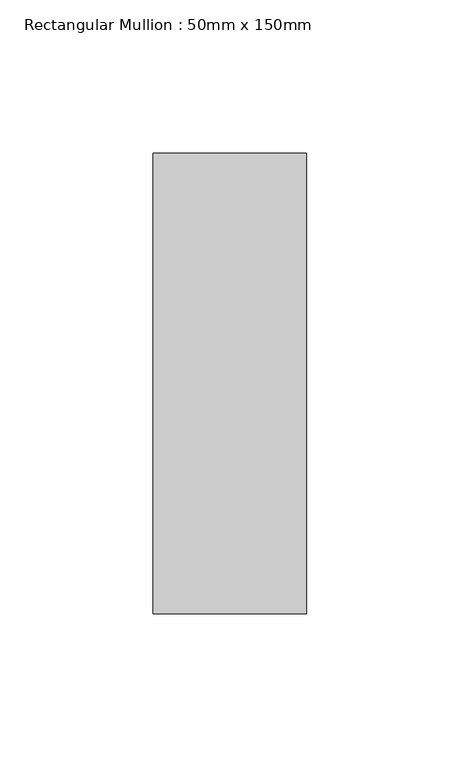
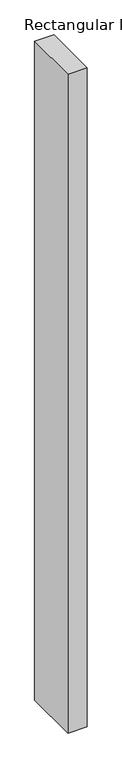
"""IFC4 building model written with IfcOpenShell, lengths in millimetres: member geometry, Rectangular Mullion : 50mm x 150mm."""

from ifc_helpers import new_model, si_unit, frame, origin, place, context, project, spatial, polyline, outline, extrude, source, transform, mapped, element, save


def rectangular_mullion_50mm_x_150mm_3f4b231f(model_context):
    return source(origin(), model_context, "Body", "SweptSolid", [
        extrude(outline(polyline([(0.0, 75.0), (0.0, -75.0), (-50.0, -75.0), (-50.0, 75.0), (0.0, 75.0)])), frame((0.0, 0.0, -1822.3836314), z_axis=(0.0, 0.0, 1.0), x_axis=(1.0, 0.0, 0.0)), (0.0, 0.0, 1.0), 1822.3836314),
    ])


if __name__ == "__main__":
    model = new_model("IFC4")
    model_context = context("Model", 3, world=origin())
    ifc_project = project(units=[si_unit("LENGTHUNIT", "METRE", prefix="MILLI")], contexts=[model_context])
    site = spatial("IfcSite", under=ifc_project)
    building = spatial("IfcBuilding", under=site)
    placement = place(None, origin())
    rectangular_mullion_50mm_x_150mm_shape = rectangular_mullion_50mm_x_150mm_3f4b231f(model_context)
    element("IfcMember", 1, ObjectType="Rectangular Mullion : 50mm x 150mm", at=placement, inside=building, context=model_context, shape_type="MappedRepresentation", body=[
        mapped(rectangular_mullion_50mm_x_150mm_shape, transform((0.0, 0.0, 0.0), x_axis=(1.0, 0.0, 0.0), y_axis=(0.0, 1.0, 0.0), z_axis=(0.0, 0.0, 1.0))),
    ])
    save(model, "model.ifc")

# Revit data of these elements
# Type "Rectangular Mullion : 50mm x 150mm"
#   built-in parameter 1007304 = 0.492126 (stored number, unit not read)
#   built-in parameter 1007301 = 0.082021 (stored number, unit not read)
#   built-in parameter 1007300 = 0.082021 (stored number, unit not read)
# Element 1 (IfcMember, "Rectangular Mullion : 50mm x 150mm")
#   Materials on its faces: "Aluminum"
# Materials
#   "Aluminum": class "Metal", colour RGB 244 244 244, transparency 0, Description = "Aluminum 6061", Cost = 0
